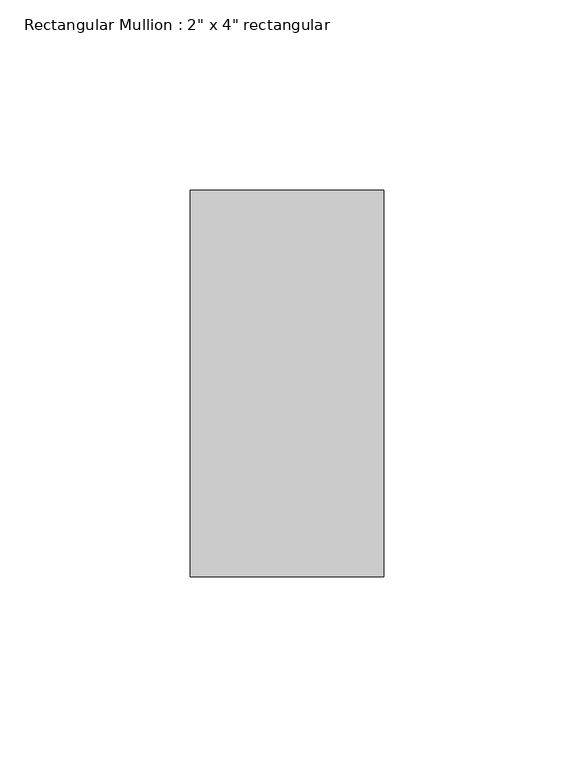
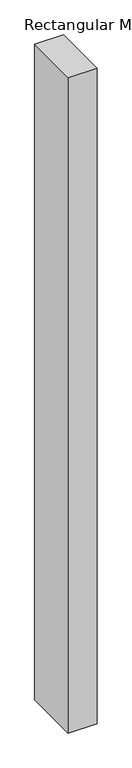
"""IFC4 building model written with IfcOpenShell, lengths in millimetres: member geometry."""

from ifc_helpers import new_model, si_unit, frame, origin, place, context, project, spatial, polyline, outline, extrude, source, transform, mapped, element, save


def member_307e65d4(model_context):
    return source(origin(), model_context, "Body", "SweptSolid", [
        extrude(outline(polyline([(25.4, 50.8), (25.4, -50.8), (-25.4, -50.8), (-25.4, 50.8), (25.4, 50.8)])), frame((0.0, 0.0, -1219.2), z_axis=(0.0, 0.0, 1.0), x_axis=(1.0, 0.0, 0.0)), (0.0, 0.0, 1.0), 1219.2),
    ])


if __name__ == "__main__":
    model = new_model("IFC4")
    model_context = context("Model", 3, world=origin())
    ifc_project = project(units=[si_unit("LENGTHUNIT", "METRE", prefix="MILLI")], contexts=[model_context])
    site = spatial("IfcSite", under=ifc_project)
    building = spatial("IfcBuilding", under=site)
    placement = place(None, origin())
    member_shape = member_307e65d4(model_context)
    element("IfcMember", 1, ObjectType="Rectangular Mullion : 2\" x 4\" rectangular", at=placement, inside=building, context=model_context, shape_type="MappedRepresentation", body=[
        mapped(member_shape, transform((0.0, 0.0, 0.0), x_axis=(1.0, 0.0, 0.0), y_axis=(0.0, 1.0, 0.0), z_axis=(0.0, 0.0, 1.0))),
    ])
    save(model, "model.ifc")

# Revit data of these elements
# Type "Rectangular Mullion : 2\" x 4\" rectangular"
#   built-in parameter 1007304 = 0.333333 (stored number, unit not read)
#   built-in parameter 1007301 = 0.0833333 (stored number, unit not read)
#   built-in parameter 1007300 = 0.0833333 (stored number, unit not read)
